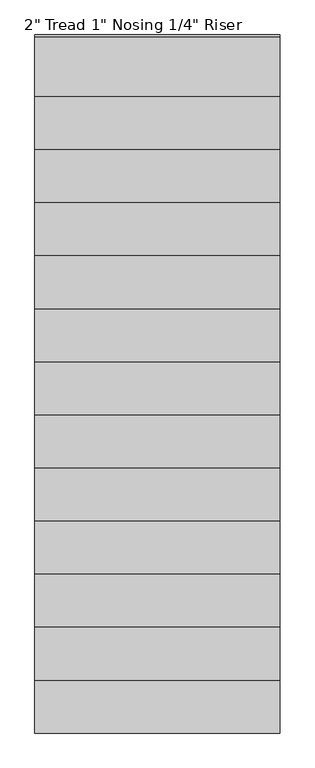
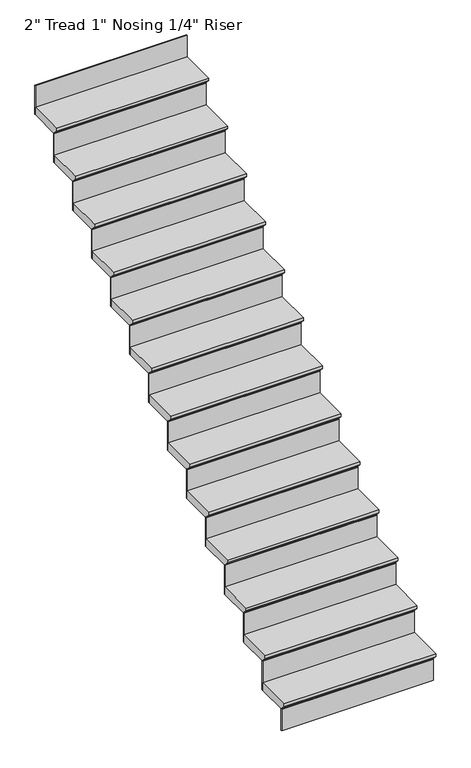
"""IFC4 building model written with IfcOpenShell, lengths in millimetres: stair flight geometry."""

from ifc_helpers import new_model, si_unit, frame, origin, place, context, project, spatial, polyline, outline, extrude, source, transform, mapped, element, save


def stair_flight_b746b64e(model_context):
    return source(origin(), model_context, "Body", "SweptSolid", [
        extrude(outline(polyline([(-2791.5111242, -2476.5), (-2562.9111242, -2476.5), (-2562.9111242, -2527.3), (-2766.1111242, -2527.3), (-2766.1111242, -2520.95), (-2791.5111242, -2495.55), (-2791.5111242, -2476.5)])), frame((-2052.1803068, 0.0, 0.0), z_axis=(1.0, 0.0, 0.0), x_axis=(0.0, 1.0, 0.0)), (0.0, 0.0, 1.0), 939.8),
        extrude(outline(polyline([(-1112.3803068, -2759.7611242), (-1112.3803068, -2766.1111242), (-2052.1803068, -2766.1111242), (-2052.1803068, -2759.7611242), (-1112.3803068, -2759.7611242)])), frame((0.0, 0.0, -2667.0), z_axis=(0.0, 0.0, 1.0), x_axis=(1.0, 0.0, 0.0)), (0.0, 0.0, 1.0), 139.7),
        extrude(outline(polyline([(-1112.3803068, -2556.5611242), (-1112.3803068, -2562.9111242), (-2052.1803068, -2562.9111242), (-2052.1803068, -2556.5611242), (-1112.3803068, -2556.5611242)])), frame((0.0, 0.0, -2527.3), z_axis=(0.0, 0.0, 1.0), x_axis=(1.0, 0.0, 0.0)), (0.0, 0.0, 1.0), 190.5),
        extrude(outline(polyline([(-2588.3111242, -2286.0), (-2359.7111242, -2286.0), (-2359.7111242, -2336.8), (-2562.9111242, -2336.8), (-2562.9111242, -2330.45), (-2588.3111242, -2305.05), (-2588.3111242, -2286.0)])), frame((-2052.1803068, 0.0, 0.0), z_axis=(1.0, 0.0, 0.0), x_axis=(0.0, 1.0, 0.0)), (0.0, 0.0, 1.0), 939.8),
        extrude(outline(polyline([(-1112.3803068, -2353.3611242), (-1112.3803068, -2359.7111242), (-2052.1803068, -2359.7111242), (-2052.1803068, -2353.3611242), (-1112.3803068, -2353.3611242)])), frame((0.0, 0.0, -2336.8), z_axis=(0.0, 0.0, 1.0), x_axis=(1.0, 0.0, 0.0)), (0.0, 0.0, 1.0), 190.5),
        extrude(outline(polyline([(-2385.1111242, -2095.5), (-2156.5111242, -2095.5), (-2156.5111242, -2146.3), (-2359.7111242, -2146.3), (-2359.7111242, -2139.95), (-2385.1111242, -2114.55), (-2385.1111242, -2095.5)])), frame((-2052.1803068, 0.0, 0.0), z_axis=(1.0, 0.0, 0.0), x_axis=(0.0, 1.0, 0.0)), (0.0, 0.0, 1.0), 939.8),
        extrude(outline(polyline([(-1112.3803068, -2150.1611242), (-1112.3803068, -2156.5111242), (-2052.1803068, -2156.5111242), (-2052.1803068, -2150.1611242), (-1112.3803068, -2150.1611242)])), frame((0.0, 0.0, -2146.3), z_axis=(0.0, 0.0, 1.0), x_axis=(1.0, 0.0, 0.0)), (0.0, 0.0, 1.0), 190.5),
        extrude(outline(polyline([(-2181.9111242, -1905.0), (-1953.3111242, -1905.0), (-1953.3111242, -1955.8), (-2156.5111242, -1955.8), (-2156.5111242, -1949.45), (-2181.9111242, -1924.05), (-2181.9111242, -1905.0)])), frame((-2052.1803068, 0.0, 0.0), z_axis=(1.0, 0.0, 0.0), x_axis=(0.0, 1.0, 0.0)), (0.0, 0.0, 1.0), 939.8),
        extrude(outline(polyline([(-1112.3803068, -1946.9611242), (-1112.3803068, -1953.3111242), (-2052.1803068, -1953.3111242), (-2052.1803068, -1946.9611242), (-1112.3803068, -1946.9611242)])), frame((0.0, 0.0, -1955.8), z_axis=(0.0, 0.0, 1.0), x_axis=(1.0, 0.0, 0.0)), (0.0, 0.0, 1.0), 190.5),
        extrude(outline(polyline([(-1978.7111242, -1714.5), (-1750.1111242, -1714.5), (-1750.1111242, -1765.3), (-1953.3111242, -1765.3), (-1953.3111242, -1758.95), (-1978.7111242, -1733.55), (-1978.7111242, -1714.5)])), frame((-2052.1803068, 0.0, 0.0), z_axis=(1.0, 0.0, 0.0), x_axis=(0.0, 1.0, 0.0)), (0.0, 0.0, 1.0), 939.8),
        extrude(outline(polyline([(-1112.3803068, -1743.7611242), (-1112.3803068, -1750.1111242), (-2052.1803068, -1750.1111242), (-2052.1803068, -1743.7611242), (-1112.3803068, -1743.7611242)])), frame((0.0, 0.0, -1765.3), z_axis=(0.0, 0.0, 1.0), x_axis=(1.0, 0.0, 0.0)), (0.0, 0.0, 1.0), 190.5),
        extrude(outline(polyline([(-1775.5111242, -1524.0), (-1546.9111242, -1524.0), (-1546.9111242, -1574.8), (-1750.1111242, -1574.8), (-1750.1111242, -1568.45), (-1775.5111242, -1543.05), (-1775.5111242, -1524.0)])), frame((-2052.1803068, 0.0, 0.0), z_axis=(1.0, 0.0, 0.0), x_axis=(0.0, 1.0, 0.0)), (0.0, 0.0, 1.0), 939.8),
        extrude(outline(polyline([(-1112.3803068, -1540.5611242), (-1112.3803068, -1546.9111242), (-2052.1803068, -1546.9111242), (-2052.1803068, -1540.5611242), (-1112.3803068, -1540.5611242)])), frame((0.0, 0.0, -1574.8), z_axis=(0.0, 0.0, 1.0), x_axis=(1.0, 0.0, 0.0)), (0.0, 0.0, 1.0), 190.5),
        extrude(outline(polyline([(-1572.3111242, -1333.5), (-1343.7111242, -1333.5), (-1343.7111242, -1384.3), (-1546.9111242, -1384.3), (-1546.9111242, -1377.95), (-1572.3111242, -1352.55), (-1572.3111242, -1333.5)])), frame((-2052.1803068, 0.0, 0.0), z_axis=(1.0, 0.0, 0.0), x_axis=(0.0, 1.0, 0.0)), (0.0, 0.0, 1.0), 939.8),
        extrude(outline(polyline([(-1112.3803068, -1337.3611242), (-1112.3803068, -1343.7111242), (-2052.1803068, -1343.7111242), (-2052.1803068, -1337.3611242), (-1112.3803068, -1337.3611242)])), frame((0.0, 0.0, -1384.3), z_axis=(0.0, 0.0, 1.0), x_axis=(1.0, 0.0, 0.0)), (0.0, 0.0, 1.0), 190.5),
        extrude(outline(polyline([(-1369.1111242, -1143.0), (-1140.5111242, -1143.0), (-1140.5111242, -1193.8), (-1343.7111242, -1193.8), (-1343.7111242, -1187.45), (-1369.1111242, -1162.05), (-1369.1111242, -1143.0)])), frame((-2052.1803068, 0.0, 0.0), z_axis=(1.0, 0.0, 0.0), x_axis=(0.0, 1.0, 0.0)), (0.0, 0.0, 1.0), 939.8),
        extrude(outline(polyline([(-1112.3803068, -1134.1611242), (-1112.3803068, -1140.5111242), (-2052.1803068, -1140.5111242), (-2052.1803068, -1134.1611242), (-1112.3803068, -1134.1611242)])), frame((0.0, 0.0, -1193.8), z_axis=(0.0, 0.0, 1.0), x_axis=(1.0, 0.0, 0.0)), (0.0, 0.0, 1.0), 190.5),
        extrude(outline(polyline([(-1165.9111242, -952.5), (-937.3111242, -952.5), (-937.3111242, -1003.3), (-1140.5111242, -1003.3), (-1140.5111242, -996.95), (-1165.9111242, -971.55), (-1165.9111242, -952.5)])), frame((-2052.1803068, 0.0, 0.0), z_axis=(1.0, 0.0, 0.0), x_axis=(0.0, 1.0, 0.0)), (0.0, 0.0, 1.0), 939.8),
        extrude(outline(polyline([(-1112.3803068, -930.9611242), (-1112.3803068, -937.3111242), (-2052.1803068, -937.3111242), (-2052.1803068, -930.9611242), (-1112.3803068, -930.9611242)])), frame((0.0, 0.0, -1003.3), z_axis=(0.0, 0.0, 1.0), x_axis=(1.0, 0.0, 0.0)), (0.0, 0.0, 1.0), 190.5),
        extrude(outline(polyline([(-962.7111242, -762.0), (-734.1111242, -762.0), (-734.1111242, -812.8), (-937.3111242, -812.8), (-937.3111242, -806.45), (-962.7111242, -781.05), (-962.7111242, -762.0)])), frame((-2052.1803068, 0.0, 0.0), z_axis=(1.0, 0.0, 0.0), x_axis=(0.0, 1.0, 0.0)), (0.0, 0.0, 1.0), 939.8),
        extrude(outline(polyline([(-1112.3803068, -727.7611242), (-1112.3803068, -734.1111242), (-2052.1803068, -734.1111242), (-2052.1803068, -727.7611242), (-1112.3803068, -727.7611242)])), frame((0.0, 0.0, -812.8), z_axis=(0.0, 0.0, 1.0), x_axis=(1.0, 0.0, 0.0)), (0.0, 0.0, 1.0), 190.5),
        extrude(outline(polyline([(-759.5111242, -571.5), (-530.9111242, -571.5), (-530.9111242, -622.3), (-734.1111242, -622.3), (-734.1111242, -615.95), (-759.5111242, -590.55), (-759.5111242, -571.5)])), frame((-2052.1803068, 0.0, 0.0), z_axis=(1.0, 0.0, 0.0), x_axis=(0.0, 1.0, 0.0)), (0.0, 0.0, 1.0), 939.8),
        extrude(outline(polyline([(-1112.3803068, -524.5611242), (-1112.3803068, -530.9111242), (-2052.1803068, -530.9111242), (-2052.1803068, -524.5611242), (-1112.3803068, -524.5611242)])), frame((0.0, 0.0, -622.3), z_axis=(0.0, 0.0, 1.0), x_axis=(1.0, 0.0, 0.0)), (0.0, 0.0, 1.0), 190.5),
        extrude(outline(polyline([(-556.3111242, -381.0), (-327.7111242, -381.0), (-327.7111242, -431.8), (-530.9111242, -431.8), (-530.9111242, -425.45), (-556.3111242, -400.05), (-556.3111242, -381.0)])), frame((-2052.1803068, 0.0, 0.0), z_axis=(1.0, 0.0, 0.0), x_axis=(0.0, 1.0, 0.0)), (0.0, 0.0, 1.0), 939.8),
        extrude(outline(polyline([(-1112.3803068, -321.3611242), (-1112.3803068, -327.7111242), (-2052.1803068, -327.7111242), (-2052.1803068, -321.3611242), (-1112.3803068, -321.3611242)])), frame((0.0, 0.0, -431.8), z_axis=(0.0, 0.0, 1.0), x_axis=(1.0, 0.0, 0.0)), (0.0, 0.0, 1.0), 190.5),
        extrude(outline(polyline([(-353.1111242, -190.5), (-124.5111242, -190.5), (-124.5111242, -241.3), (-327.7111242, -241.3), (-327.7111242, -234.95), (-353.1111242, -209.55), (-353.1111242, -190.5)])), frame((-2052.1803068, 0.0, 0.0), z_axis=(1.0, 0.0, 0.0), x_axis=(0.0, 1.0, 0.0)), (0.0, 0.0, 1.0), 939.8),
        extrude(outline(polyline([(-1112.3803068, -118.1611242), (-1112.3803068, -124.5111242), (-2052.1803068, -124.5111242), (-2052.1803068, -118.1611242), (-1112.3803068, -118.1611242)])), frame((0.0, 0.0, -241.3), z_axis=(0.0, 0.0, 1.0), x_axis=(1.0, 0.0, 0.0)), (0.0, 0.0, 1.0), 190.5),
    ])


if __name__ == "__main__":
    model = new_model("IFC4")
    model_context = context("Model", 3, world=origin())
    ifc_project = project(units=[si_unit("LENGTHUNIT", "METRE", prefix="MILLI")], contexts=[model_context])
    site = spatial("IfcSite", under=ifc_project)
    building = spatial("IfcBuilding", under=site)
    placement = place(None, origin())
    stair_flight_shape = stair_flight_b746b64e(model_context)
    element("IfcStairFlight", 1, ObjectType="2\" Tread 1\" Nosing 1/4\" Riser", at=placement, inside=building, context=model_context, shape_type="MappedRepresentation", body=[
        mapped(stair_flight_shape, transform((0.0, 0.0, 0.0), x_axis=(1.0, 0.0, 0.0), y_axis=(0.0, 1.0, 0.0), z_axis=(0.0, 0.0, 1.0))),
    ])
    save(model, "model.ifc")
